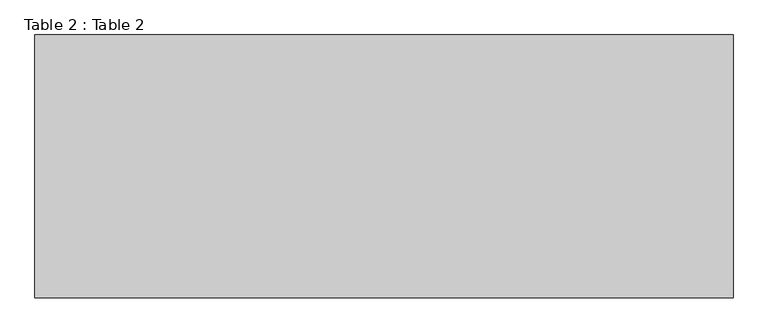
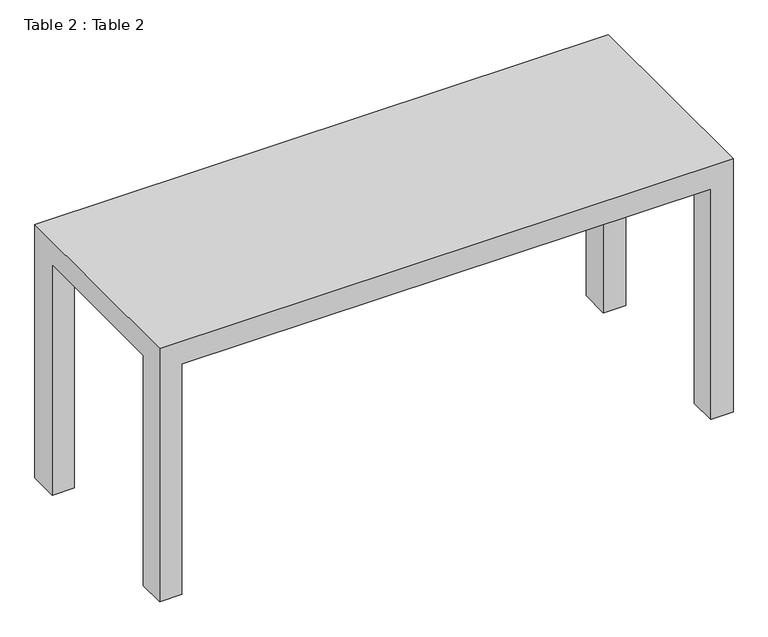
"""IFC4 building model written with IfcOpenShell, lengths in millimetres: furniture geometry, Table 2 : Table 2."""

from ifc_helpers import new_model, si_unit, origin, place, context, project, spatial, faceted_brep, source, transform, mapped, element, save


def table_2_table_2_da86e92d(model_context):
    return source(origin(), model_context, "Body", "Brep", [
        faceted_brep([(15671.7186033, 8365.6045137, 914.4), (13715.9186033, 8365.6045137, 914.4), (13715.9186033, 7629.0045137, 914.4), (15671.7186033, 7629.0045137, 914.4), (13792.1186033, 7629.0045137, 0.0), (13715.9186033, 7629.0045137, 0.0), (13715.9186033, 7725.2253688, 0.0), (13792.1186033, 7725.2253688, 0.0), (15671.7186033, 7629.0045137, 0.0), (15595.5186033, 7629.0045137, 0.0), (15595.5186033, 7725.2253688, 0.0), (15671.7186033, 7725.2253688, 0.0), (13715.9186033, 8365.6045137, 0.0), (13792.1186033, 8365.6045137, 0.0), (13792.1186033, 8264.0045137, 0.0), (13715.9186033, 8264.0045137, 0.0), (15595.5186033, 8365.6045137, 0.0), (15671.7186033, 8365.6045137, 0.0), (15671.7186033, 8264.0045137, 0.0), (15595.5186033, 8264.0045137, 0.0), (15595.5186033, 8365.6045137, 831.1593056), (13792.1186033, 8365.6045137, 831.1593056), (13715.9186033, 8264.0045137, 831.1593056), (13715.9186033, 7725.2253688, 831.1593056), (13792.1186033, 7629.0045137, 831.1593056), (15595.5186033, 7629.0045137, 831.1593056), (15671.7186033, 7725.2253688, 831.1593056), (15671.7186033, 8264.0045137, 831.1593056), (15595.5186033, 8264.0045137, 831.1593056), (15595.5186033, 7725.2253688, 831.1593056), (13792.1186033, 7725.2253688, 831.1593056), (13792.1186033, 8264.0045137, 831.1593056)], [[[0, 1, 2, 3]], [[4, 5, 6, 7]], [[8, 9, 10, 11]], [[12, 13, 14, 15]], [[16, 17, 18, 19]], [[1, 0, 17, 16, 20, 21, 13, 12]], [[2, 1, 12, 15, 22, 23, 6, 5]], [[3, 2, 5, 4, 24, 25, 9, 8]], [[0, 3, 8, 11, 26, 27, 18, 17]], [[21, 20, 28, 27, 26, 29, 25, 24, 30, 23, 22, 31]], [[13, 21, 31, 14]], [[24, 4, 7, 30]], [[20, 16, 19, 28]], [[9, 25, 29, 10]], [[31, 22, 15, 14]], [[23, 30, 7, 6]], [[27, 28, 19, 18]], [[29, 26, 11, 10]]]),
    ])


if __name__ == "__main__":
    model = new_model("IFC4")
    model_context = context("Model", 3, world=origin())
    ifc_project = project(units=[si_unit("LENGTHUNIT", "METRE", prefix="MILLI")], contexts=[model_context])
    site = spatial("IfcSite", under=ifc_project)
    building = spatial("IfcBuilding", under=site)
    placement = place(None, origin())
    table_2_table_2_shape = table_2_table_2_da86e92d(model_context)
    element("IfcFurniture", 1, ObjectType="Table 2 : Table 2", at=placement, inside=building, context=model_context, shape_type="MappedRepresentation", body=[
        mapped(table_2_table_2_shape, transform((0.0, 0.0, 0.0), x_axis=(1.0, 0.0, 0.0), y_axis=(0.0, 1.0, 0.0), z_axis=(0.0, 0.0, 1.0))),
    ])
    save(model, "model.ifc")

# Revit data of these elements
# Element 1 (IfcFurniture, "Table 2 : Table 2")
#   Materials on its faces: "food"
# Materials
#   "food": class "Glass", colour RGB 233 233 233, transparency 0, Description = "Soda Lime Glass", Cost = 0
